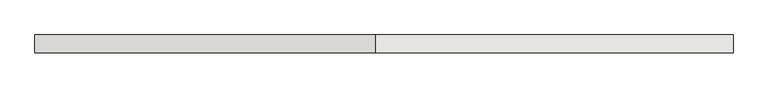
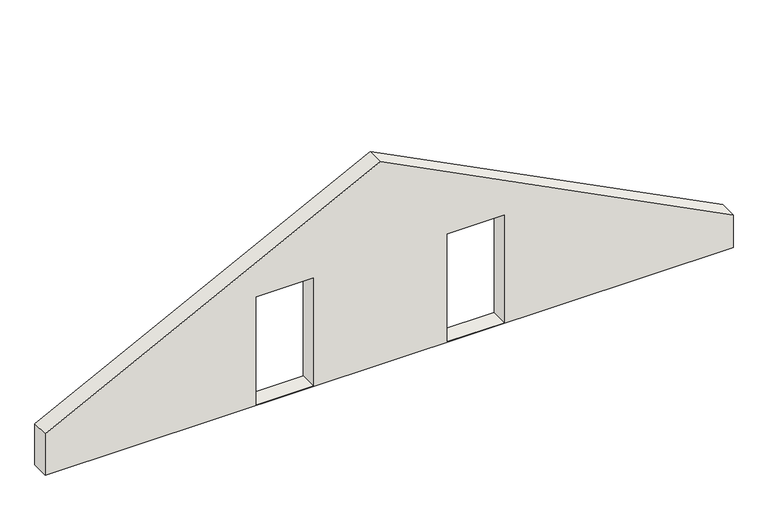
"""IFC4 building model written with IfcOpenShell, lengths in millimetres: wall geometry, 0_3d_modell."""

from ifc_helpers import new_model, si_unit, frame, origin, place, context, project, spatial, polyline, outline, extrude, source, transform, mapped, element, save


def wall_68174385(model_context):
    return source(origin(), model_context, "Body", "SweptSolid", [
        extrude(outline(polyline([(4251.6781465, 6650.0), (863.3339073, 0.0), (0.0, 0.0), (0.0, 13650.0), (685.0, 13650.0), (4251.6781465, 6650.0)]), holes=[polyline([(10.0, 7975.0), (2270.0, 7975.0), (2270.0, 9110.0), (10.0, 9110.0), (10.0, 7975.0)]), polyline([(10.0, 4190.0), (2270.0, 4190.0), (2270.0, 5325.0), (10.0, 5325.0), (10.0, 4190.0)])]), frame((0.0, 0.0, 0.0), z_axis=(0.0, 1.0, 0.0), x_axis=(0.0, 0.0, 1.0)), (0.0, 0.0, 1.0), 350.0),
    ])


if __name__ == "__main__":
    model = new_model("IFC4")
    model_context = context("Model", 3, world=origin())
    ifc_project = project(units=[si_unit("LENGTHUNIT", "METRE", prefix="MILLI")], contexts=[model_context])
    site = spatial("IfcSite", under=ifc_project)
    building = spatial("IfcBuilding", under=site)
    placement = place(None, origin())
    wall_shape = wall_68174385(model_context)
    element("IfcWall", 1, ObjectType="0_3d_modell", at=placement, inside=building, context=model_context, shape_type="MappedRepresentation", body=[
        mapped(wall_shape, transform((0.0, 0.0, 0.0), x_axis=(1.0, 0.0, 0.0), y_axis=(0.0, 1.0, 0.0), z_axis=(0.0, 0.0, 1.0))),
    ])
    save(model, "model.ifc")

# Revit data of these elements
# Element 1 (IfcWall, "0_3d_modell")
#   Materials on its faces: "holzschalung"
# Materials
#   "holzschalung": class "Unassigned", colour RGB 128 128 128, transparency 0
